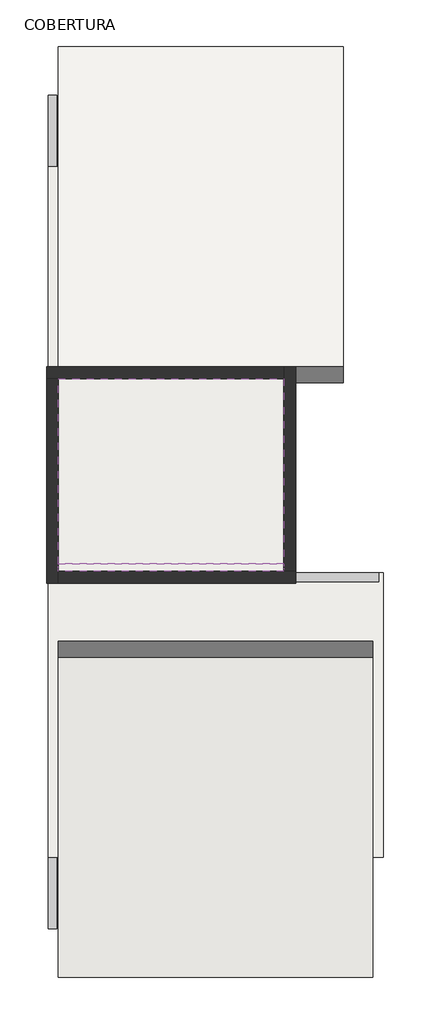
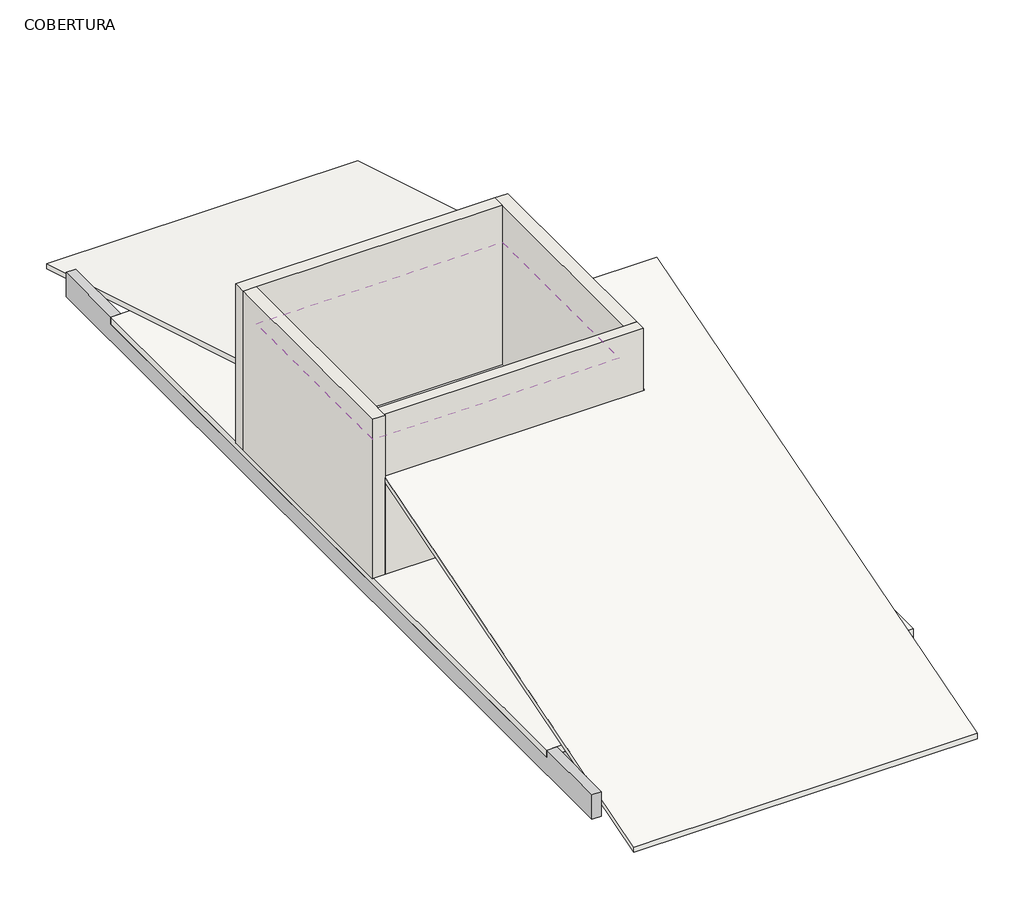
# One storey: 8 beams, 4 walls, 3 roofs, 1 pipe segment, 1 slab.
"""IFC4 building model written with IfcOpenShell, lengths in millimetres."""

from ifc_helpers import new_model, si_unit, frame, origin, place, context, project, spatial, polyline, outline, extrude, faceted_brep, element, save

model = new_model("IFC4")

# Units and contexts
model_context = context("Model", 3, world=origin())
ifc_project = project(units=[si_unit("LENGTHUNIT", "METRE", prefix="MILLI")], contexts=[model_context])

# Site, building, storey
site = spatial("IfcSite", under=ifc_project)
building = spatial("IfcBuilding", under=site)
storey = spatial("IfcBuildingStorey", under=building, Name="COBERTURA", Elevation=6160.0)

# Beams
placement = place(None, origin())
element("IfcBeam", 1, ObjectType="Concreto-Viga retangular : VIGA 15 x 40 cm", at=placement, inside=storey, context=model_context, shape_type="Brep", body=[
    faceted_brep([(-2693.4017601, -7116.8729018, 6160.0), (-2843.4017601, -7116.8729018, 6160.0), (-2843.4017601, -7116.8729018, 5760.0), (-2693.4017601, -7116.8729018, 5760.0), (-2693.4017601, 6933.1270982, 6160.0), (-2693.4017601, 6933.1270982, 5760.0), (-2843.4017601, 6933.1270982, 5760.0), (-2843.4017601, 6933.1270982, 6160.0), (-2693.4017601, -5916.8729018, 6160.0), (-2843.4017601, -5916.8729018, 6160.0), (-2843.4017601, -5916.8729018, 6040.0), (-2843.4017601, 5733.1270982, 6040.0), (-2843.4017601, 5733.1270982, 6160.0), (-2693.4017601, 5733.1270982, 5760.0), (-2693.4017601, 5583.1270982, 5760.0), (-2693.4017601, 882.7270982, 5760.0), (-2693.4017601, 732.7270982, 5760.0), (-2693.4017601, -5766.8729018, 5760.0), (-2693.4017601, -5916.8729018, 5760.0), (-2693.4017601, 5733.1270982, 6160.0), (-2693.4017601, 5733.1270982, 6040.0), (-2693.4017601, 5583.1270982, 6040.0), (-2693.4017601, 882.7270982, 6040.0), (-2693.4017601, 732.7270982, 6040.0), (-2693.4017601, -5766.8729018, 6040.0), (-2693.4017601, -5916.8729018, 6040.0)], [[[0, 1, 2, 3]], [[4, 5, 6, 7]], [[1, 0, 8, 9]], [[2, 1, 9, 10, 11, 12, 7, 6]], [[3, 2, 6, 5, 13, 14, 15, 16, 17, 18]], [[0, 3, 18, 17, 16, 15, 14, 13, 5, 4, 19, 20, 21, 22, 23, 24, 25, 8]], [[10, 25, 24, 23, 22, 21, 20, 11]], [[11, 20, 19, 12]], [[25, 10, 9, 8]], [[4, 7, 12, 19]]]),
])
element("IfcBeam", 2, ObjectType="Concreto-Viga retangular : VIGA 15 x 40 cm", at=placement, inside=storey, context=model_context, shape_type="Brep", body=[
    faceted_brep([(1306.5982399, 5733.1270982, 5760.0), (1131.5982399, 5733.1270982, 5760.0), (-2668.4017601, 5733.1270982, 5760.0), (-2693.4017601, 5733.1270982, 5760.0), (-2693.4017601, 5733.1270982, 6040.0), (1306.5982399, 5733.1270982, 6040.0), (-2693.4017601, 5583.1270982, 5760.0), (1306.5982399, 5583.1270982, 5760.0), (1156.5982399, 5583.1270982, 5760.0), (1131.5982399, 5583.1270982, 5760.0), (-2668.4017601, 5583.1270982, 5760.0), (1306.5982399, 5583.1270982, 6040.0), (1156.5982399, 5583.1270982, 6040.0), (1131.5982399, 5583.1270982, 6040.0), (-2668.4017601, 5583.1270982, 6040.0), (-2693.4017601, 5583.1270982, 6040.0)], [[[0, 1, 2, 3, 4, 5]], [[6, 3, 2, 1, 0, 7, 8, 9, 10]], [[6, 10, 9, 8, 7, 11, 12, 13, 14, 15]], [[3, 6, 15, 4]], [[7, 0, 5, 11]], [[5, 4, 15, 14, 13, 12, 11]]]),
])
element("IfcBeam", 3, ObjectType="Concreto-Viga retangular : VIGA 15 x 40 cm", at=placement, inside=storey, context=model_context, shape_type="Brep", body=[
    faceted_brep([(2806.5982399, -1191.8729018, 5760.0), (2656.5982399, -1191.8729018, 5760.0), (2656.5982399, -1191.8729018, 6040.0), (2806.5982399, -1191.8729018, 6040.0), (2806.5982399, -5916.8729018, 5760.0), (2806.5982399, -5916.8729018, 6040.0), (2656.5982399, -5916.8729018, 5760.0), (2656.5982399, -5766.8729018, 5760.0), (2656.5982399, -5916.8729018, 6040.0), (2656.5982399, -5766.8729018, 6040.0)], [[[0, 1, 2, 3]], [[4, 0, 3, 5]], [[1, 0, 4, 6, 7]], [[1, 7, 6, 8, 9, 2]], [[6, 4, 5, 8]], [[3, 2, 9, 8, 5]]]),
])
element("IfcBeam", 4, ObjectType="Concreto-Viga retangular : VIGA 15 x 40 cm", at=placement, inside=storey, context=model_context, shape_type="Brep", body=[
    faceted_brep([(1156.5982399, 882.7270982, 5760.0), (1131.5982399, 882.7270982, 5760.0), (-1668.4017601, 882.7270982, 5760.0), (-2693.4017601, 882.7270982, 5760.0), (-2693.4017601, 882.7270982, 6040.0), (-1668.4017601, 882.7270982, 6040.0), (1131.5982399, 882.7270982, 6040.0), (1156.5982399, 882.7270982, 6040.0), (-2693.4017601, 732.7270982, 5760.0), (1156.5982399, 732.7270982, 5760.0), (1131.5982399, 732.7270982, 5760.0), (-1668.4017601, 732.7270982, 5760.0), (1156.5982399, 732.7270982, 6040.0), (1131.5982399, 732.7270982, 6040.0), (-1668.4017601, 732.7270982, 6040.0), (-2693.4017601, 732.7270982, 6040.0)], [[[0, 1, 2, 3, 4, 5, 6, 7]], [[8, 3, 2, 1, 0, 9, 10, 11]], [[8, 11, 10, 9, 12, 13, 14, 15]], [[3, 8, 15, 4]], [[9, 0, 7, 12]], [[7, 6, 5, 4, 15, 14, 13, 12]]]),
])
element("IfcBeam", 5, ObjectType="Concreto-Viga retangular : VIGA 15 x 40 cm", at=placement, inside=storey, context=model_context, shape_type="Brep", body=[
    faceted_brep([(-2768.4017601, -1266.8729018, 6560.0), (-2768.4017601, -1116.8729018, 6560.0), (-2768.4017601, -1116.8729018, 6160.0), (-2768.4017601, -1266.8729018, 6160.0), (2731.5982399, -1266.8729018, 6560.0), (2731.5982399, -1266.8729018, 6160.0), (2731.5982399, -1116.8729018, 6160.0), (2731.5982399, -1116.8729018, 6560.0), (-2668.4017601, -1266.8729018, 6560.0), (1331.5982399, -1266.8729018, 6560.0), (2631.5982399, -1266.8729018, 6560.0), (2631.5982399, -1116.8729018, 6560.0), (1331.5982399, -1116.8729018, 6560.0), (-2668.4017601, -1116.8729018, 6560.0), (1331.5982399, -1116.8729018, 6160.0), (1306.5982399, -1116.8729018, 6160.0), (-2668.4017601, -1116.8729018, 6160.0), (2631.5982399, -1266.8729018, 6160.0), (1331.5982399, -1266.8729018, 6160.0), (-2668.4017601, -1266.8729018, 6160.0)], [[[0, 1, 2, 3]], [[4, 5, 6, 7]], [[1, 0, 8, 9, 10, 4, 7, 11, 12, 13]], [[2, 1, 13, 12, 11, 7, 6, 14, 15, 16]], [[3, 2, 16, 15, 14, 6, 5, 17, 18, 19]], [[0, 3, 19, 18, 17, 5, 4, 10, 9, 8]]]),
])
element("IfcBeam", 6, ObjectType="Concreto-Viga retangular : VIGA 15 x 40 cm", at=placement, inside=storey, context=model_context, shape_type="Brep", body=[
    faceted_brep([(-2693.4017601, -5916.8729018, 5760.0), (-2668.4017601, -5916.8729018, 5760.0), (2631.5982399, -5916.8729018, 5760.0), (2656.5982399, -5916.8729018, 5760.0), (2656.5982399, -5916.8729018, 6040.0), (-2693.4017601, -5916.8729018, 6040.0), (2656.5982399, -5766.8729018, 5760.0), (-2693.4017601, -5766.8729018, 5760.0), (-2668.4017601, -5766.8729018, 5760.0), (2631.5982399, -5766.8729018, 5760.0), (-2693.4017601, -5766.8729018, 6040.0), (-2668.4017601, -5766.8729018, 6040.0), (2631.5982399, -5766.8729018, 6040.0), (2656.5982399, -5766.8729018, 6040.0)], [[[0, 1, 2, 3, 4, 5]], [[6, 3, 2, 1, 0, 7, 8, 9]], [[6, 9, 8, 7, 10, 11, 12, 13]], [[3, 6, 13, 4]], [[7, 0, 5, 10]], [[5, 4, 13, 12, 11, 10]]]),
])
element("IfcBeam", 7, ObjectType="Concreto-Viga retangular : VIGA 15 x 40 cm", at=placement, inside=storey, context=model_context, shape_type="Brep", body=[
    faceted_brep([(1156.5982399, -1091.8729018, 5760.0), (1306.5982399, -1091.8729018, 5760.0), (1306.5982399, -1091.8729018, 6040.0), (1156.5982399, -1091.8729018, 6040.0), (1306.5982399, 5583.1270982, 5760.0), (1306.5982399, 5583.1270982, 6040.0), (1156.5982399, 732.7270982, 5760.0), (1156.5982399, 882.7270982, 5760.0), (1156.5982399, 5583.1270982, 5760.0), (1156.5982399, 732.7270982, 6040.0), (1156.5982399, 882.7270982, 6040.0), (1156.5982399, 5583.1270982, 6040.0)], [[[0, 1, 2, 3]], [[1, 4, 5, 2]], [[1, 0, 6, 7, 8, 4]], [[8, 7, 6, 0, 3, 9, 10, 11]], [[4, 8, 11, 5]], [[3, 2, 5, 11, 10, 9]]]),
])
element("IfcBeam", 8, ObjectType="Concreto-Viga retangular : VIGA 15 x 40 cm", at=placement, inside=storey, context=model_context, shape_type="Brep", body=[
    faceted_brep([(-2768.4017601, 2183.3918499, 6560.0), (-2768.4017601, 2333.3918499, 6560.0), (-2768.4017601, 2333.3918499, 6160.0), (-2768.4017601, 2183.3918499, 6160.0), (1231.5982399, 2183.3918499, 6560.0), (1231.5982399, 2183.3918499, 6160.0), (1231.5982399, 2333.3918499, 6160.0), (1231.5982399, 2333.3918499, 6560.0), (1131.5982399, 2183.3918499, 6560.0), (1131.5982399, 2333.3918499, 6560.0), (1131.5982399, 2333.3918499, 6160.0), (1131.5982399, 2183.3918499, 6160.0)], [[[0, 1, 2, 3]], [[4, 5, 6, 7]], [[1, 0, 8, 4, 7, 9]], [[2, 1, 9, 7, 6, 10]], [[3, 2, 10, 6, 5, 11]], [[0, 3, 11, 5, 4, 8]]]),
])

# Pipe segment
element("IfcPipeSegment", 9, ObjectType=".CALHA 12.5 cm", at=placement, inside=storey, context=model_context, shape_type="SweptSolid", body=[
    extrude(outline(polyline([(-966.8729018, 8115.4867724), (-1041.0729018, 8115.4867724), (-1079.1729018, 8214.999005), (-1091.8729018, 8214.999005), (-1091.8729018, 8227.699005), (-1079.1729018, 8227.699005), (-1079.1729018, 8224.524005), (-1088.6979018, 8224.524005), (-1088.6979018, 8218.174005), (-1076.8106044, 8218.174005), (-1038.7106044, 8118.6617724), (-970.0479018, 8118.6617724), (-970.0479018, 8240.399005), (-966.8729018, 8240.399005), (-966.8729018, 8115.4867724)])), frame((-2668.4017601, 0.0, 0.0), z_axis=(1.0, 0.0, 0.0), x_axis=(0.0, 1.0, 0.0)), (0.0, 0.0, 1.0), 3800.0),
])

# Roofs
element("IfcRoof", 10, ObjectType="TELHA METÁLICA", at=placement, inside=storey, context=model_context, shape_type="SweptSolid", body=[
    extrude(outline(polyline([(-966.8729018, 8240.399005), (2158.3918499, 8552.9254801), (2158.3918499, 8472.5264752), (-966.8729018, 8160.0), (-966.8729018, 8240.399005)])), frame((-2668.4017601, 0.0, 0.0), z_axis=(1.0, 0.0, 0.0), x_axis=(0.0, 1.0, 0.0)), (0.0, 0.0, 1.0), 3800.0),
])
element("IfcRoof", 11, ObjectType=".TELHA CERÂMICA", at=placement, inside=storey, context=model_context, shape_type="Brep", body=[
    faceted_brep([(1331.5982399, 2358.3918499, 7279.9205745), (-2668.4017601, 2358.3918499, 7279.9205745), (-2668.4017601, 7758.1270982, 5660.0), (2131.5982399, 7758.1270982, 5660.0), (2131.5982399, 1558.3918499, 7519.9205745), (1331.5982399, 1558.3918499, 7519.9205745), (-2668.4017601, 2358.3918499, 7363.4430266), (1331.5982399, 2358.3918499, 7363.4430266), (1331.5982399, 1558.3918499, 7603.4430266), (2131.5982399, 1558.3918499, 7603.4430266), (2131.5982399, 7758.1270982, 5743.5224521), (-2668.4017601, 7758.1270982, 5743.5224521)], [[[0, 1, 2, 3, 4, 5]], [[6, 7, 8, 9, 10, 11]], [[2, 11, 10, 3]], [[7, 6, 1, 0]], [[6, 11, 2, 1]], [[10, 9, 4, 3]], [[9, 8, 5, 4]], [[8, 7, 0, 5]]]),
])
element("IfcRoof", 12, ObjectType=".TELHA CERÂMICA", at=placement, inside=storey, context=model_context, shape_type="Brep", body=[
    faceted_brep([(-2668.4017601, -1266.8729018, 7662.5), (1351.5982399, -1266.8729018, 7662.5), (1351.5982399, 628.4235797, 8231.0889444), (2631.5982399, 628.4235797, 8231.0889444), (2631.5982399, -7941.8729018, 5660.0), (-2668.4017601, -7941.8729018, 5660.0), (1351.5982399, -1266.8729018, 7746.0224521), (-2668.4017601, -1266.8729018, 7746.0224521), (-2668.4017601, -7941.8729018, 5743.5224521), (2631.5982399, -7941.8729018, 5743.5224521), (2631.5982399, 628.4235797, 8314.6113965), (1351.5982399, 628.4235797, 8314.6113965)], [[[0, 1, 2, 3, 4, 5]], [[6, 7, 8, 9, 10, 11]], [[4, 9, 8, 5]], [[7, 6, 1, 0]], [[8, 7, 0, 5]], [[10, 9, 4, 3]], [[11, 10, 3, 2]], [[6, 11, 2, 1]]]),
])

# Slab
element("IfcSlab", 13, ObjectType=".EST. LAJE 12 cm - CONCRETO", at=placement, inside=storey, context=model_context, shape_type="Brep", body=[
    faceted_brep([(-2843.4017601, 5733.1270982, 6040.0), (-2693.4017601, 5733.1270982, 6040.0), (-2668.4017601, 5733.1270982, 6040.0), (1131.5982399, 5733.1270982, 6040.0), (1156.5982399, 5733.1270982, 6040.0), (1306.5982399, 5733.1270982, 6040.0), (1306.5982399, 5583.1270982, 6040.0), (1306.5982399, -1091.8729018, 6040.0), (1306.5982399, -1116.8729018, 6040.0), (2631.5982399, -1116.8729018, 6040.0), (2806.5982399, -1116.8729018, 6040.0), (2806.5982399, -1191.8729018, 6040.0), (2806.5982399, -5916.8729018, 6040.0), (2656.5982399, -5916.8729018, 6040.0), (2631.5982399, -5916.8729018, 6040.0), (-2668.4017601, -5916.8729018, 6040.0), (-2693.4017601, -5916.8729018, 6040.0), (-2843.4017601, -5916.8729018, 6040.0), (-2843.4017601, 5733.1270982, 6160.0), (-2843.4017601, 2358.3918499, 6160.0), (-2843.4017601, -1291.8729018, 6160.0), (-2843.4017601, -5916.8729018, 6160.0), (-2693.4017601, -5916.8729018, 6160.0), (-2668.4017601, -5916.8729018, 6160.0), (2631.5982399, -5916.8729018, 6160.0), (2806.5982399, -5916.8729018, 6160.0), (2806.5982399, -1116.8729018, 6160.0), (2731.5982399, -1116.8729018, 6160.0), (2631.5982399, -1116.8729018, 6160.0), (1351.5982399, -1116.8729018, 6160.0), (1306.5982399, -1116.8729018, 6160.0), (1306.5982399, -1091.8729018, 6160.0), (1306.5982399, 2358.3918499, 6160.0), (1306.5982399, 5733.1270982, 6160.0), (1131.5982399, 5733.1270982, 6160.0), (-2668.4017601, 5733.1270982, 6160.0), (-2693.4017601, 5733.1270982, 6160.0)], [[[0, 1, 2, 3, 4, 5, 6, 7, 8, 9, 10, 11, 12, 13, 14, 15, 16, 17]], [[18, 19, 20, 21, 22, 23, 24, 25, 26, 27, 28, 29, 30, 31, 32, 33, 34, 35, 36]], [[5, 4, 3, 2, 1, 0, 18, 36, 35, 34, 33]], [[8, 7, 6, 5, 33, 32, 31, 30]], [[10, 9, 8, 30, 29, 28, 27, 26]], [[12, 11, 10, 26, 25]], [[17, 16, 15, 14, 13, 12, 25, 24, 23, 22, 21]], [[0, 17, 21, 20, 19, 18]]]),
])

# Walls
element("IfcWall", 14, ObjectType=".EXT. PAREDE 20 cm - PINTURA/PINTURA", at=placement, inside=storey, context=model_context, shape_type="Brep", body=[
    faceted_brep([(-2868.4017601, 2158.3918499, 6160.0), (-2668.4017601, 2158.3918499, 6160.0), (1131.5982399, 2158.3918499, 6160.0), (1131.5982399, 2158.3918499, 8760.0), (-2668.4017601, 2158.3918499, 8760.0), (-2868.4017601, 2158.3918499, 8760.0), (-2868.4017601, 2358.3918499, 8760.0), (1131.5982399, 2358.3918499, 8760.0), (1131.5982399, 2358.3918499, 6160.0), (-2668.4017601, 2358.3918499, 6160.0), (-2868.4017601, 2358.3918499, 6160.0), (-2868.4017601, 2358.3918499, 7542.8874906), (1131.5982399, 2183.3918499, 6160.0), (1131.5982399, 2183.3918499, 6560.0), (1131.5982399, 2333.3918499, 6560.0), (1131.5982399, 2333.3918499, 6160.0), (-2868.4017601, 2333.3918499, 6160.0), (-2768.4017601, 2333.3918499, 6160.0), (-2768.4017601, 2183.3918499, 6160.0), (-2768.4017601, 2333.3918499, 6560.0), (-2768.4017601, 2183.3918499, 6560.0)], [[[0, 1, 2, 3, 4, 5]], [[6, 7, 8, 9, 10, 11]], [[5, 4, 3, 7, 6]], [[3, 2, 12, 13, 14, 15, 8, 7]], [[5, 6, 11, 10, 16, 0]], [[2, 1, 0, 16, 17, 18, 12]], [[16, 10, 9, 8, 15, 17]], [[19, 20, 18, 17]], [[20, 19, 14, 13]], [[19, 17, 15, 14]], [[18, 20, 13, 12]]]),
])
element("IfcWall", 15, ObjectType=".EXT. PAREDE 20 cm - PINTURA/PINTURA", at=placement, inside=storey, context=model_context, shape_type="Brep", body=[
    faceted_brep([(-2668.4017601, -1291.8729018, 6160.0), (-2668.4017601, -1091.8729018, 6160.0), (-2668.4017601, 2158.3918499, 6160.0), (-2668.4017601, 2158.3918499, 8760.0), (-2668.4017601, -1091.8729018, 8760.0), (-2668.4017601, -1266.8729018, 8760.0), (-2668.4017601, -1291.8729018, 8760.0), (-2668.4017601, -1291.8729018, 7917.8327839), (-2668.4017601, -1291.8729018, 7655.0), (-2868.4017601, -1291.8729018, 8760.0), (-2868.4017601, 2158.3918499, 8760.0), (-2868.4017601, 2158.3918499, 6160.0), (-2868.4017601, -1291.8729018, 6160.0), (-2868.4017601, -1291.8729018, 7917.8327839), (-2843.4017601, -1291.8729018, 6160.0), (-2843.4017601, 2158.3918499, 6160.0)], [[[0, 1, 2, 3, 4, 5, 6, 7, 8]], [[9, 10, 11, 12, 13]], [[6, 5, 4, 3, 10, 9]], [[6, 9, 13, 12, 14, 0, 8, 7]], [[10, 3, 2, 15, 11]], [[2, 1, 0, 14, 15]], [[14, 12, 11, 15]]]),
])
element("IfcWall", 16, ObjectType=".EXT. PAREDE 20 cm - PINTURA/PINTURA", at=placement, inside=storey, context=model_context, shape_type="Brep", body=[
    faceted_brep([(1331.5982399, -1091.8729018, 6160.0), (1131.5982399, -1091.8729018, 6160.0), (-2668.4017601, -1091.8729018, 6160.0), (-2668.4017601, -1091.8729018, 8760.0), (1131.5982399, -1091.8729018, 8760.0), (1331.5982399, -1091.8729018, 8760.0), (1331.5982399, -1291.8729018, 6160.0), (1331.5982399, -1291.8729018, 7655.0), (-2668.4017601, -1291.8729018, 7655.0), (-2668.4017601, -1291.8729018, 6160.0), (1331.5982399, -1266.8729018, 8760.0), (1331.5982399, -1266.8729018, 7662.5), (1331.5982399, -1266.8729018, 6160.0), (1331.5982399, -1266.8729018, 6560.0), (1331.5982399, -1116.8729018, 6560.0), (1331.5982399, -1116.8729018, 6160.0), (-2668.4017601, -1116.8729018, 6160.0), (-2668.4017601, -1116.8729018, 6560.0), (-2668.4017601, -1266.8729018, 6560.0), (-2668.4017601, -1266.8729018, 6160.0), (-2668.4017601, -1266.8729018, 7662.5), (-2668.4017601, -1266.8729018, 8760.0)], [[[0, 1, 2, 3, 4, 5]], [[6, 7, 8, 9]], [[0, 5, 10, 11, 7, 6, 12, 13, 14, 15]], [[3, 2, 16, 17, 18, 19, 9, 8, 20, 21]], [[2, 1, 0, 15, 16]], [[12, 6, 9, 19]], [[13, 18, 17, 14]], [[14, 17, 16, 15]], [[18, 13, 12, 19]], [[5, 4, 3, 21, 10]], [[10, 21, 20, 11]], [[20, 8, 7, 11]]]),
])
element("IfcWall", 17, ObjectType=".EXT. PAREDE 20 cm - PINTURA/PINTURA", at=placement, inside=storey, context=model_context, shape_type="Brep", body=[
    faceted_brep([(1131.5982399, 2358.3918499, 6160.0), (1131.5982399, 2333.3918499, 6160.0), (1131.5982399, 2183.3918499, 6160.0), (1131.5982399, 2158.3918499, 6160.0), (1131.5982399, -1091.8729018, 6160.0), (1131.5982399, -1091.8729018, 8760.0), (1131.5982399, 2158.3918499, 8760.0), (1131.5982399, 2358.3918499, 8760.0), (1131.5982399, 2358.3918499, 7279.9205745), (1331.5982399, 2358.3918499, 6160.0), (1331.5982399, 2358.3918499, 7279.9205745), (1331.5982399, 2358.3918499, 8760.0), (1331.5982399, -1091.8729018, 8760.0), (1331.5982399, -1091.8729018, 6160.0), (1306.5982399, 2358.3918499, 6160.0), (1306.5982399, -1091.8729018, 6160.0)], [[[0, 1, 2, 3, 4, 5, 6, 7, 8]], [[9, 10, 11, 12, 13]], [[7, 6, 5, 12, 11]], [[0, 8, 7, 11, 10, 9, 14]], [[5, 4, 15, 13, 12]], [[4, 3, 2, 1, 0, 14, 15]], [[14, 9, 13, 15]]]),
])

save(model, "model.ifc")

# Revit data of these elements
# Project information
#   Project Issue Date = "Data de emissão"
#   Project Status = "Status do projeto"
#   Client Name = "JOSÉ APARECIDO GARCIA"
#   Project Address = "RUA MONTE ALEGRE, LOTE 17 - QUADRA K"
#   Project Name = "CONSTRUÇÃO UNIFAMILIAR"
# Type "Concreto-Viga retangular : VIGA 15 x 40 cm"
#   Length [instance default] = 1.524 m
#   b = 0.15 m
#   h = 0.40 m
#   Structural Material [instance default] = Concreto, Moldado no local - Cinza
#   Assembly Code = ""
# Type "TELHA METÁLICA"
#   Layers, outside or top first: 0.08 m ".TELHA METÁLICA" (function 1)
# Type ".TELHA CERÂMICA"
#   Layers, outside or top first: 0.08 m ".TELHAS" (function 1)
# Type ".EST. LAJE 12 cm - CONCRETO"
#   Function = 0
#   Layers, outside or top first: 0.12 m ".CONCRETO ESTRUTURAL" (function 1)
# Type ".EXT. PAREDE 20 cm - PINTURA/PINTURA"
#   Layers, outside or top first: 0.025 m ".ARGAMASSA + PINTURA BRANCA" (function 5); 0.15 m ".ALVENARIA" (function 1); 0.025 m ".ARGAMASSA + PINTURA BRANCA" (function 5)
# Elements 1, 2, 3, 4, 5, 6, 7, 8 (IfcBeam, "Concreto-Viga retangular : VIGA 15 x 40 cm")
#   Comments = ""
#   Structural Material = .CONCRETO ESTRUTURAL
#   Phase Created = Construção nova
#   Materials on its faces: ".CONCRETO ESTRUTURAL"
# Element 9 (IfcPipeSegment, ".CALHA 12.5 cm")
#   Phase Created = Construção nova
#   Materials on its faces: ".ALUMÍNIO"
# Element 10 (IfcRoof, "TELHA METÁLICA")
#   built-in parameter 1001705 = 28.0608 (stored number, unit not read)
#   built-in parameter 1001701 = 6.56168 (stored number, unit not read)
#   built-in parameter 1001710 = 33615
#   Phase Created = Construção nova
#   Materials on its faces: ".TELHA METÁLICA"
# Element 11 (IfcRoof, ".TELHA CERÂMICA")
#   built-in parameter 1001705 = 24.9457 (stored number, unit not read)
#   built-in parameter 1001701 = -1.64042 (stored number, unit not read)
#   built-in parameter 1001710 = 33615
#   Phase Created = Construção nova
#   Materials on its faces: ".TELHAS"
# Element 12 (IfcRoof, ".TELHA CERÂMICA")
#   built-in parameter 1001705 = 27.2789 (stored number, unit not read)
#   built-in parameter 1001701 = -1.64042 (stored number, unit not read)
#   built-in parameter 1001710 = 33615
#   Phase Created = Construção nova
#   Materials on its faces: ".TELHAS"
# Element 13 (IfcSlab, ".EST. LAJE 12 cm - CONCRETO")
#   built-in parameter 1001955 = 3.14159 (stored number, unit not read)
#   Height Offset From Level = 0.00 m
#   Phase Created = Construção nova
#   Materials on its faces: ".CONCRETO ESTRUTURAL"
# Elements 14, 15, 16, 17 (IfcWall, ".EXT. PAREDE 20 cm - PINTURA/PINTURA")
#   Top Offset = 0.00 m
#   Base Offset = 0.00 m
#   Unconnected Height = 2.60 m
#   wall height = 2.60 m
#   Phase Created = Construção nova
#   Base Constraint = COBERTURA
#   Materials on its faces: "Material pré-definido de parede", ".ARGAMASSA + PINTURA BRANCA"
# Materials
#   "Concreto, Moldado no local - Cinza": class "Concreto", colour RGB 192 192 192, transparency 0, Description = "Concreto moldado no local", Cost = 0
#   ".TELHA METÁLICA": class "Genérico", colour RGB 120 120 120, transparency 0, Cost = 0
#   ".TELHAS": class "Genérico", colour RGB 134 55 46, transparency 0, Cost = 0
#   ".CONCRETO ESTRUTURAL": class "Genérico", colour RGB 155 155 155, transparency 0, Description = "Material de telhado betuminoso", Cost = 0
#   ".ARGAMASSA + PINTURA BRANCA": class "Genérico", colour RGB 255 255 255, transparency 0, Cost = 0
#   ".ALVENARIA": class "Alvenaria", colour RGB 192 192 192, transparency 0, Comments = "m²", Description = "Alvenaria em tijolo comum, bloco cerâmico ou bloco de concreto", Cost = 0
#   ".ALUMÍNIO": class "CC_METAIS", colour RGB 244 244 244, transparency 0, Description = "Material alumínio", Cost = 0
#   "Material pré-definido de parede": class "Diversos", colour RGB 128 128 128, transparency 0
